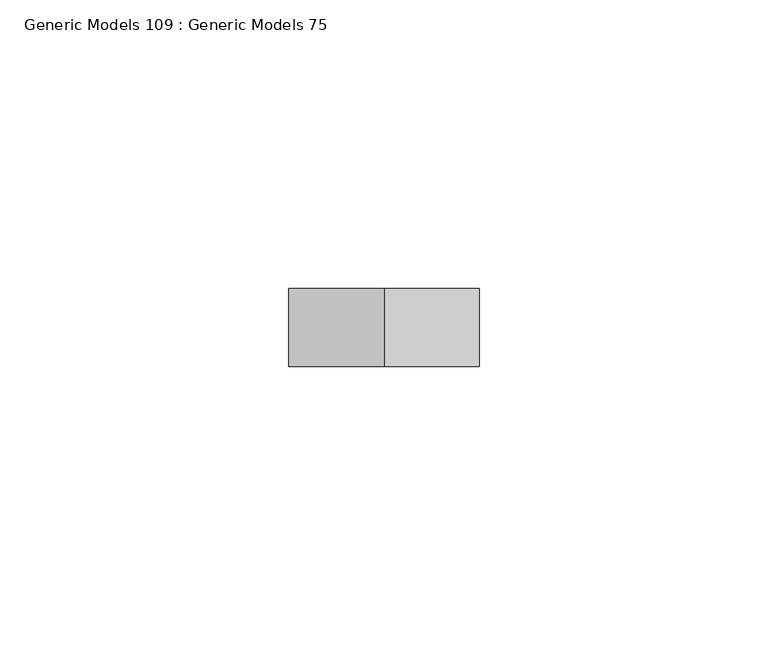
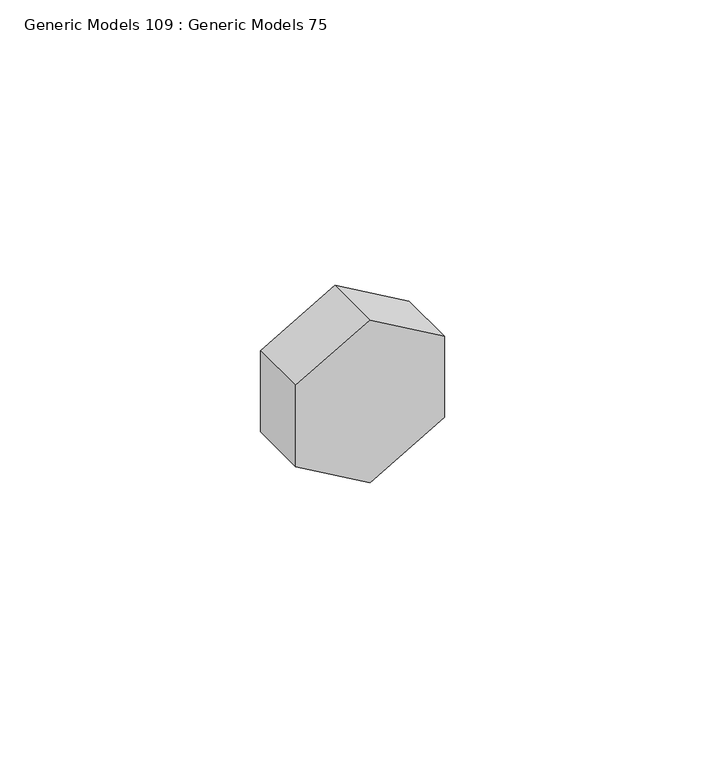
"""IFC4 building model written with IfcOpenShell, lengths in millimetres: proxy geometry, Generic Models 109 : Generic Models 75."""

from ifc_helpers import new_model, si_unit, frame, origin, place, context, project, spatial, polyline, outline, extrude, source, transform, mapped, element, save


def generic_models_109_generic_models_75_f4c88c96(model_context):
    return source(origin(), model_context, "Body", "SweptSolid", [
        extrude(outline(polyline([(268485.9375, 31991.9073871), (268504.9875, 31991.9073871), (268514.5125, 31975.4096032), (268504.9875, 31958.9118192), (268485.9375, 31958.9118192), (268476.4125, 31975.4096032), (268485.9375, 31991.9073871)])), frame((0.0, 30676.7094112, 0.0), z_axis=(0.0, 1.0, 0.0), x_axis=(0.0, 0.0, 1.0)), (0.0, 0.0, 1.0), 13.49375),
    ])


if __name__ == "__main__":
    model = new_model("IFC4")
    model_context = context("Model", 3, world=origin())
    ifc_project = project(units=[si_unit("LENGTHUNIT", "METRE", prefix="MILLI")], contexts=[model_context])
    site = spatial("IfcSite", under=ifc_project)
    building = spatial("IfcBuilding", under=site)
    placement = place(None, origin())
    generic_models_109_generic_models_75_shape = generic_models_109_generic_models_75_f4c88c96(model_context)
    element("IfcBuildingElementProxy", 1, Name="Generic Models 109 : Generic Models 75", ObjectType="Generic Models 109 : Generic Models 75", at=placement, inside=building, context=model_context, shape_type="MappedRepresentation", body=[
        mapped(generic_models_109_generic_models_75_shape, transform((0.0, 0.0, 0.0), x_axis=(1.0, 0.0, 0.0), y_axis=(0.0, 1.0, 0.0), z_axis=(0.0, 0.0, 1.0))),
    ])
    save(model, "model.ifc")
